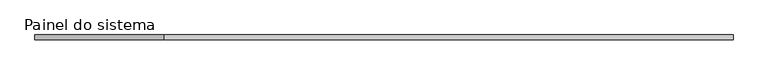
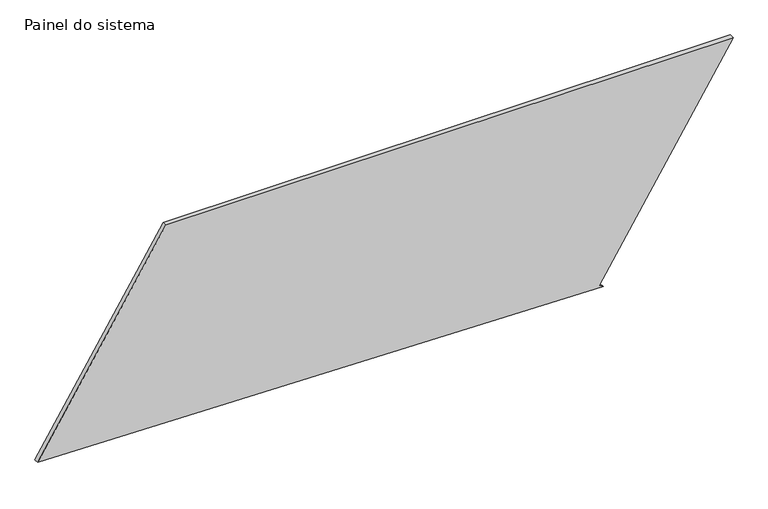
"""IFC4 building model written with IfcOpenShell, lengths in millimetres: plate geometry, Painel do sistema : Envidraçado."""

from ifc_helpers import new_model, si_unit, frame, origin, place, context, project, spatial, polyline, outline, extrude, source, transform, mapped, element, save


def painel_do_sistema_a85c4b84(model_context):
    return source(origin(), model_context, "Body", "SweptSolid", [
        extrude(outline(polyline([(0.0, 1151.3655035), (13.2016257, 1130.1354051), (1152.8993124, 1838.8397164), (1152.8993124, -1161.180471), (63.1265228, -1838.8397164), (0.0, 1151.3655035)])), frame((0.0, 24.5, 0.0), z_axis=(0.0, 1.0, 0.0), x_axis=(0.0, 0.0, 1.0)), (0.0, 0.0, 1.0), 25.0),
    ])


if __name__ == "__main__":
    model = new_model("IFC4")
    model_context = context("Model", 3, world=origin())
    ifc_project = project(units=[si_unit("LENGTHUNIT", "METRE", prefix="MILLI")], contexts=[model_context])
    site = spatial("IfcSite", under=ifc_project)
    building = spatial("IfcBuilding", under=site)
    placement = place(None, origin())
    painel_do_sistema_shape = painel_do_sistema_a85c4b84(model_context)
    element("IfcPlate", 1, ObjectType="Painel do sistema : Envidraçado", at=placement, inside=building, context=model_context, shape_type="MappedRepresentation", body=[
        mapped(painel_do_sistema_shape, transform((0.0, 0.0, 0.0), x_axis=(1.0, 0.0, 0.0), y_axis=(0.0, 1.0, 0.0), z_axis=(0.0, 0.0, 1.0))),
    ])
    save(model, "model.ifc")

# Revit data of these elements
# Type "Painel do sistema : Envidraçado"
#   Construction Type Id = "GSP4R"
#   Analytic Construction = "Vidraça única Pilkington 1/8 pol"
#   Visual Light Transmittance = 0.9
#   Solar Heat Gain Coefficient = 0.86
#   Heat Transfer Coefficient (U) = 6.7069 W/(m²·K)
# Element 1 (IfcPlate, "Painel do sistema : Envidraçado")
#   Materials on its faces: "Vidro"
# Materials
#   "Vidro": class "Vidro", colour RGB 0 128 192, transparency 0.9, Description = "Vidro de sílica", Cost = 0
